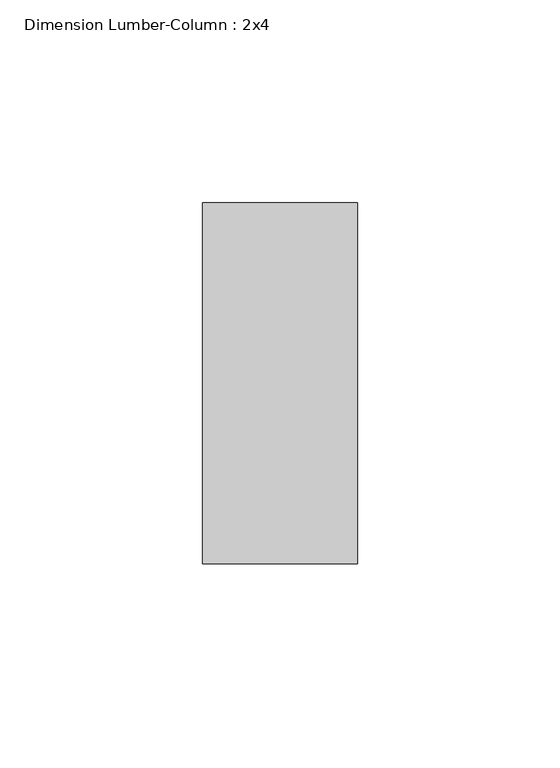
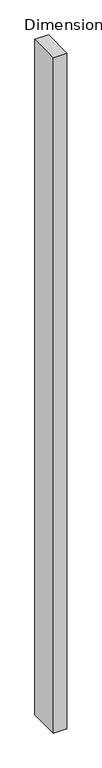
"""IFC4 building model written with IfcOpenShell, lengths in millimetres: column geometry, Dimension Lumber-Column : 2x4."""

from ifc_helpers import new_model, si_unit, frame, origin, place, context, project, spatial, polyline, outline, extrude, source, transform, mapped, element, save


def dimension_lumber_column_2x4_0f816ddf(model_context):
    return source(origin(), model_context, "Body", "SweptSolid", [
        extrude(outline(polyline([(19.05, 44.45), (19.05, -44.45), (-19.05, -44.45), (-19.05, 44.45), (19.05, 44.45)])), frame((0.0, 0.0, 56.35625), z_axis=(0.0, 0.0, 1.0), x_axis=(1.0, 0.0, 0.0)), (0.0, 0.0, 1.0), 1999.853125),
    ])


if __name__ == "__main__":
    model = new_model("IFC4")
    model_context = context("Model", 3, world=origin())
    ifc_project = project(units=[si_unit("LENGTHUNIT", "METRE", prefix="MILLI")], contexts=[model_context])
    site = spatial("IfcSite", under=ifc_project)
    building = spatial("IfcBuilding", under=site)
    placement = place(None, origin())
    dimension_lumber_column_2x4_shape = dimension_lumber_column_2x4_0f816ddf(model_context)
    element("IfcColumn", 1, ObjectType="Dimension Lumber-Column : 2x4", at=placement, inside=building, context=model_context, shape_type="MappedRepresentation", body=[
        mapped(dimension_lumber_column_2x4_shape, transform((0.0, 0.0, 0.0), x_axis=(1.0, 0.0, 0.0), y_axis=(0.0, 1.0, 0.0), z_axis=(0.0, 0.0, 1.0))),
    ])
    save(model, "model.ifc")

# Revit data of these elements
# Type "Dimension Lumber-Column : 2x4"
#   Int Type = "Interior"
#   Assembly Code = "B10"
#   Cost = 8.05
#   A = 0.0364583 SF
#   b = 0' - 1 1/2"
#   d = 0' - 3 1/2"
#   Structural Material [instance default] = Softwood, Lumber
# Element 1 (IfcColumn, "Dimension Lumber-Column : 2x4")
#   Structural Material = Douglas Fir #2
#   Materials on its faces: "Douglas Fir #2"
# Materials
#   "Softwood, Lumber": class "Wood", colour RGB 223 192 134, transparency 0, Description = "Pinus Echinata", Cost = 0
#   "Douglas Fir #2": class "Wood", colour RGB 223 192 134, transparency 0, Description = "Pinus Echinata", Cost = 0
